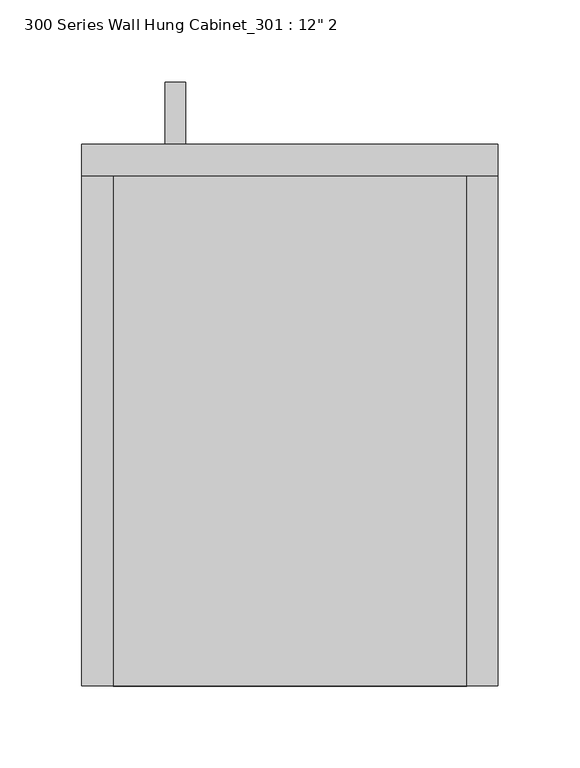
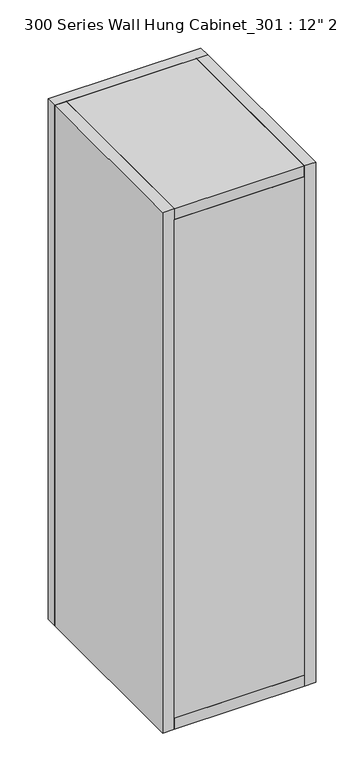
"""IFC4 building model written with IfcOpenShell, lengths in millimetres: furniture geometry."""

from ifc_helpers import new_model, si_unit, frame, origin, place, context, project, spatial, polyline, outline, extrude, source, transform, mapped, element, save


def furniture_bfdc1b7c(model_context):
    return source(origin(), model_context, "Body", "SweptSolid", [
        extrude(outline(polyline([(406.4, 1352.5425373), (406.4, 1365.2121874), (444.4810937, 1365.2121874), (444.4810937, 1270.0), (406.4, 1270.0), (406.4, 1282.6696501), (431.8114436, 1282.6696501), (431.8114436, 1352.5425373), (406.4, 1352.5425373)])), frame((-76.2, 0.0, 0.0), z_axis=(1.0, 0.0, 0.0), x_axis=(0.0, 1.0, 0.0)), (0.0, 0.0, 1.0), 12.4065288),
        extrude(outline(polyline([(107.95, 387.35), (107.95, 76.2), (-107.95, 76.2), (-107.95, 387.35), (107.95, 387.35)])), frame((0.0, 0.0, 1219.2), z_axis=(0.0, 0.0, 1.0), x_axis=(1.0, 0.0, 0.0)), (0.0, 0.0, 1.0), 19.05),
        extrude(outline(polyline([(107.95, 76.2), (-107.95, 76.2), (-107.95, 95.25), (107.95, 95.25), (107.95, 76.2)])), frame((0.0, 0.0, 1238.25), z_axis=(0.0, 0.0, 1.0), x_axis=(1.0, 0.0, 0.0)), (0.0, 0.0, 1.0), 876.3),
        extrude(outline(polyline([(127.0, 387.35), (-127.0, 387.35), (-127.0, 406.4), (127.0, 406.4), (127.0, 387.35)])), frame((0.0, 0.0, 1219.2), z_axis=(0.0, 0.0, 1.0), x_axis=(1.0, 0.0, 0.0)), (0.0, 0.0, 1.0), 914.4),
        extrude(outline(polyline([(-127.0, 76.2), (-127.0, 387.35), (-107.95, 387.35), (-107.95, 76.2), (-127.0, 76.2)])), frame((0.0, 0.0, 1219.2), z_axis=(0.0, 0.0, 1.0), x_axis=(1.0, 0.0, 0.0)), (0.0, 0.0, 1.0), 914.4),
        extrude(outline(polyline([(107.95, 76.2), (107.95, 387.35), (127.0, 387.35), (127.0, 76.2), (107.95, 76.2)])), frame((0.0, 0.0, 1219.2), z_axis=(0.0, 0.0, 1.0), x_axis=(1.0, 0.0, 0.0)), (0.0, 0.0, 1.0), 914.4),
        extrude(outline(polyline([(107.95, 387.35), (107.95, 76.2), (-107.95, 76.2), (-107.95, 387.35), (107.95, 387.35)])), frame((0.0, 0.0, 2114.55), z_axis=(0.0, 0.0, 1.0), x_axis=(1.0, 0.0, 0.0)), (0.0, 0.0, 1.0), 19.05),
    ])


if __name__ == "__main__":
    model = new_model("IFC4")
    model_context = context("Model", 3, world=origin())
    ifc_project = project(units=[si_unit("LENGTHUNIT", "METRE", prefix="MILLI")], contexts=[model_context])
    site = spatial("IfcSite", under=ifc_project)
    building = spatial("IfcBuilding", under=site)
    placement = place(None, origin())
    furniture_shape = furniture_bfdc1b7c(model_context)
    element("IfcFurniture", 1, ObjectType="300 Series Wall Hung Cabinet_301 : 12\" 2", at=placement, inside=building, context=model_context, shape_type="MappedRepresentation", body=[
        mapped(furniture_shape, transform((0.0, 0.0, 0.0), x_axis=(1.0, 0.0, 0.0), y_axis=(0.0, 1.0, 0.0), z_axis=(0.0, 0.0, 1.0))),
    ])
    save(model, "model.ifc")

# Revit data of these elements
# Type "300 Series Wall Hung Cabinet_301 : 12\" 2"
#   URL = "www.wicnet.org/manual_sections.asp"
#   Model = "301"
#   Manufacturer = "Woodwork Institute"
#   Description = "Wall Hung Cabinet"
#   Content Creator URL = "www.AECcontent.com"
#   Content Creator = "AECcontent"
#   Assembly Code = "E2010200"
#   Width = 0' - 10"
#   Top of Cabinet = 7' - 0"
#   Height = 3' - 0"
#   Depth = 1' - 1"
#   Top Panel Material = Cabinet
#   Side Panel Material = Cabinet
#   Door Panel Material = Cabinet
#   Shelf Panel Material = Cabinet
# Element 1 (IfcFurniture, "300 Series Wall Hung Cabinet_301 : 12\" 2")
#   Materials on its faces: "Cabinet", "Default metal"
# Materials
#   "Cabinet": class "Wood", colour RGB 189 170 130, transparency 0, Cost = 0
#   "Default metal": class "Unassigned", colour RGB 204 204 204, transparency 0
